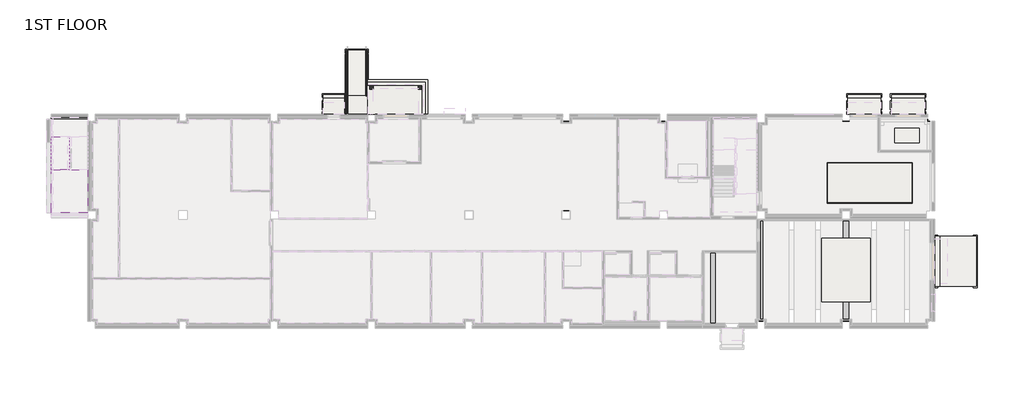
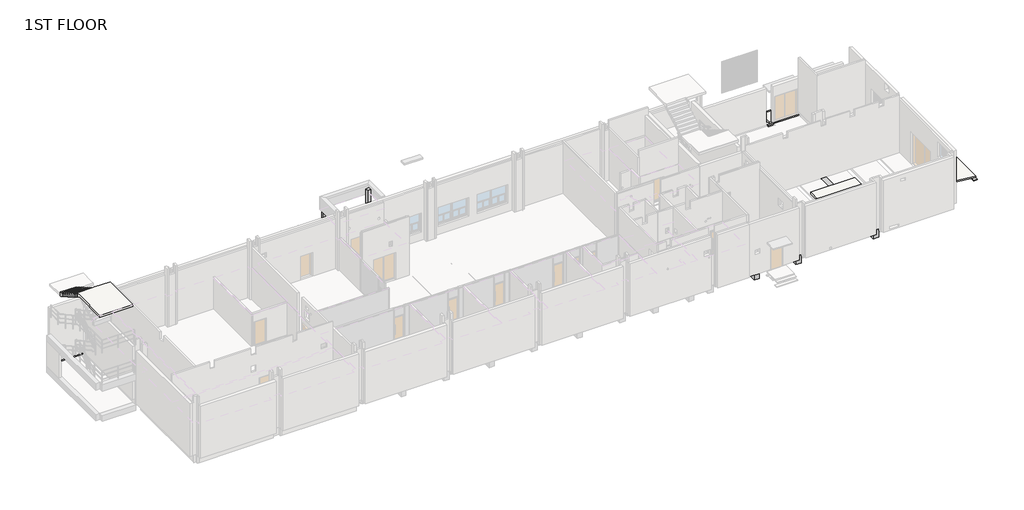
# One storey, part 10 of 15: 37 slabs, 9 beams, 2 columns, 1 stair flight.
"""IFC4 building model written with IfcOpenShell, lengths in millimetres."""

from ifc_helpers import new_model, si_unit, frame, origin, place, context, project, spatial, polyline, outline, extrude, faceted_brep, element, save

model = new_model("IFC4")

# Units and contexts
model_context = context("Model", 3, world=origin())
ifc_project = project(units=[si_unit("LENGTHUNIT", "METRE", prefix="MILLI")], contexts=[model_context])

# Site, building, storey
site = spatial("IfcSite", under=ifc_project)
building = spatial("IfcBuilding", under=site)
storey = spatial("IfcBuildingStorey", under=building, Name="1ST FLOOR", Elevation=4800.0)

# Beams
placement = place(None, origin())
element("IfcBeam", 1, ObjectType="RC Beam_Rectangular : H_SB_AR S16_TG-UG_500x800_1G2A", at=placement, inside=storey, context=model_context, shape_type="Brep", body=[
    faceted_brep([(50825.0, -7850.0, 4800.0), (47350.0, -7850.0, 4800.0), (47350.0, -8350.0, 4800.0), (50825.0, -8350.0, 4800.0), (47350.0, -8350.0, 4650.0), (47350.0, -8350.0, 4000.0), (50825.0, -8350.0, 4000.0), (50825.0, -8350.0, 4650.0), (47350.0, -7850.0, 4000.0), (50825.0, -7850.0, 4000.0), (50825.0, -7850.0, 4650.0), (47350.0, -7850.0, 4650.0)], [[[0, 1, 2, 3]], [[3, 2, 4, 5, 6, 7]], [[8, 9, 6, 5]], [[1, 0, 10, 9, 8, 11]], [[0, 3, 7, 6, 9, 10]], [[8, 5, 4, 2, 1, 11]]]),
])
element("IfcBeam", 2, ObjectType="RC Beam_Rectangular : H_SB_AR S16_TG-UG_500x800_1G1", at=placement, inside=storey, context=model_context, shape_type="Brep", body=[
    faceted_brep([(38750.0, -300.0, 4800.0), (38750.0, -7650.0, 4800.0), (39250.0, -7650.0, 4800.0), (39250.0, -300.0, 4800.0), (39250.0, -7650.0, 4650.0), (39250.0, -7650.0, 4000.0), (39250.0, -300.0, 4000.0), (39250.0, -300.0, 4650.0), (38750.0, -7650.0, 4000.0), (38750.0, -300.0, 4000.0), (38750.0, -300.0, 4650.0), (38750.0, -7650.0, 4650.0)], [[[0, 1, 2, 3]], [[3, 2, 4, 5, 6, 7]], [[6, 5, 8, 9]], [[1, 0, 10, 9, 8, 11]], [[8, 5, 4, 2, 1, 11]], [[0, 3, 7, 6, 9, 10]]]),
])
element("IfcBeam", 3, ObjectType="RC Beam_Rectangular : H_SB_AR S16_TG-UG_500x800_1G1", at=placement, inside=storey, context=model_context, shape_type="Brep", body=[
    faceted_brep([(46800.0, -300.0, 4800.0), (46800.0, -7650.0, 4800.0), (47300.0, -7650.0, 4800.0), (47300.0, -4975.0, 4800.0), (47300.0, -4825.0, 4800.0), (47300.0, -300.0, 4800.0), (47150.0, -300.0, 4800.0), (47300.0, -7650.0, 4000.0), (47300.0, -300.0, 4000.0), (47300.0, -7650.0, 4650.0), (46800.0, -7650.0, 4000.0), (46800.0, -300.0, 4000.0), (46800.0, -300.0, 4650.0), (46800.0, -7650.0, 4650.0)], [[[0, 1, 2, 3, 4, 5, 6]], [[7, 8, 5, 4, 3, 2, 9]], [[8, 7, 10, 11]], [[1, 0, 12, 11, 10, 13]], [[0, 6, 5, 8, 11, 12]], [[10, 7, 9, 2, 1, 13]]]),
])
element("IfcBeam", 4, ObjectType="RC Beam_Rectangular : H_SB_AR S16_TG-UG_450x800_1B1", at=placement, inside=storey, context=model_context, shape_type="Brep", body=[
    faceted_brep([(42125.0, -100.0, 4800.0), (41675.0, -100.0, 4800.0), (41675.0, -7850.0, 4800.0), (42125.0, -7850.0, 4800.0), (42125.0, -7850.0, 4650.0), (42125.0, -7850.0, 4000.0), (42125.0, -100.0, 4000.0), (42125.0, -100.0, 4650.0), (41675.0, -100.0, 4000.0), (41675.0, -7850.0, 4000.0), (41675.0, -100.0, 4650.0), (41675.0, -7850.0, 4650.0)], [[[0, 1, 2, 3]], [[0, 3, 4, 5, 6, 7]], [[8, 6, 5, 9]], [[2, 1, 10, 8, 9, 11]], [[1, 0, 7, 6, 8, 10]], [[3, 2, 11, 9, 5, 4]]]),
])
element("IfcBeam", 5, ObjectType="RC Beam_Rectangular : H_SB_AR S16_TG-UG_450x800_1B1", at=placement, inside=storey, context=model_context, shape_type="Brep", body=[
    faceted_brep([(45325.0, -100.0, 4800.0), (44875.0, -100.0, 4800.0), (44875.0, -7850.0, 4800.0), (45325.0, -7850.0, 4800.0), (45325.0, -7850.0, 4650.0), (45325.0, -7850.0, 4000.0), (45325.0, -100.0, 4000.0), (45325.0, -100.0, 4650.0), (44875.0, -100.0, 4000.0), (44875.0, -7850.0, 4000.0), (44875.0, -100.0, 4650.0), (44875.0, -7850.0, 4650.0)], [[[0, 1, 2, 3]], [[0, 3, 4, 5, 6, 7]], [[8, 6, 5, 9]], [[2, 1, 10, 8, 9, 11]], [[1, 0, 7, 6, 8, 10]], [[3, 2, 11, 9, 5, 4]]]),
])
element("IfcBeam", 6, ObjectType="RC Beam_Rectangular : H_SB_AR S16_TG-UG_450x800_1B1A", at=placement, inside=storey, context=model_context, shape_type="Brep", body=[
    faceted_brep([(50825.0, -8350.0, 4800.0), (51275.0, -8350.0, 4800.0), (51275.0, -8350.0, 4650.0), (51275.0, -8350.0, 4000.0), (50825.0, -8350.0, 4000.0), (50825.0, -8350.0, 4650.0), (50825.0, -16900.0, 4800.0), (51275.0, -16900.0, 4800.0), (51275.0, -16900.0, 4650.0), (51275.0, -16900.0, 4000.0), (50825.0, -16900.0, 4000.0), (50825.0, -15750.0000001, 4000.0), (50825.0, -16900.0, 4650.0)], [[[0, 1, 2, 3, 4, 5]], [[1, 0, 6, 7]], [[1, 7, 8, 9, 3, 2]], [[4, 3, 9, 10, 11]], [[6, 0, 5, 4, 11, 10, 12]], [[7, 6, 12, 10, 9, 8]]]),
])
element("IfcBeam", 7, ObjectType="RC Beam_Rectangular : H_SB_AR S16_TG-UG_500x800_1G1", at=placement, inside=storey, context=model_context, shape_type="Brep", body=[
    faceted_brep([(54700.0, -8350.0, 4800.0), (54700.0, -16700.0, 4800.0), (55200.0, -16700.0, 4800.0), (55200.0, -8350.0, 4800.0), (55200.0, -16700.0, 4650.0), (55200.0, -16700.0, 4000.0), (55200.0, -8350.0, 4000.0), (55200.0, -8350.0, 4650.0), (54700.0, -16700.0, 4000.0), (54700.0, -8350.0, 4000.0), (54700.0, -8350.0, 4650.0), (54700.0, -16700.0, 4650.0)], [[[0, 1, 2, 3]], [[3, 2, 4, 5, 6, 7]], [[6, 5, 8, 9]], [[1, 0, 10, 9, 8, 11]], [[0, 3, 7, 6, 9, 10]], [[8, 5, 4, 2, 1, 11]]]),
])
element("IfcBeam", 8, ObjectType="RC Beam_Rectangular : H_SB_AR S16_TG-UG_500x800_1G1", at=placement, inside=storey, context=model_context, shape_type="Brep", body=[
    faceted_brep([(61750.0, -8350.0, 4800.0), (61750.0, -16700.0, 4800.0), (62250.0, -16700.0, 4800.0), (62250.0, -8350.0, 4800.0), (62250.0, -16700.0, 4650.0), (62250.0, -16700.0, 4000.0), (62250.0, -8350.0, 4000.0), (62250.0, -8350.0, 4650.0), (61750.0, -16700.0, 4000.0), (61750.0, -8350.0, 4000.0), (61750.0, -8350.0, 4650.0), (61750.0, -16700.0, 4650.0)], [[[0, 1, 2, 3]], [[3, 2, 4, 5, 6, 7]], [[6, 5, 8, 9]], [[1, 0, 10, 9, 8, 11]], [[0, 3, 7, 6, 9, 10]], [[8, 5, 4, 2, 1, 11]]]),
])
element("IfcBeam", 9, ObjectType="RC Beam_Rectangular : H_SB_AR S16_RC Beam-AG_400x530_SG1A", at=placement, inside=storey, context=model_context, shape_type="Brep", body=[
    faceted_brep([(-300.0, -100.0, 4630.0), (-300.0, 50.0, 4630.0), (-300.0, 300.0, 4630.0), (-3300.0, 300.0, 4630.0), (-3300.0, 50.0, 4630.0), (-3300.0, -100.0, 4630.0), (-300.0, -100.0, 4100.0), (-300.0, -100.0, 4430.0), (-3300.0, -100.0, 4430.0), (-3300.0, -100.0, 4100.0), (-300.0, 300.0, 4100.0), (-3300.0, 300.0, 4100.0)], [[[0, 1, 2, 3, 4, 5]], [[6, 7, 0, 5, 8, 9]], [[10, 6, 9, 11]], [[2, 10, 11, 3]], [[2, 1, 0, 7, 6, 10]], [[3, 11, 9, 8, 5, 4]]]),
])

# Columns
element("IfcColumn", 10, ObjectType="RC_Column_Rectangular : H_SC_AR S15_RC Col-AG_300x300_C4", at=placement, inside=storey, context=model_context, shape_type="Brep", body=[
    faceted_brep([(23150.0, 2650.0, 4585.0), (23150.0, 2620.0, 4585.0), (23150.0, 2350.0, 4585.0), (22850.0, 2350.0, 4585.0), (22850.0, 2620.0, 4585.0), (22850.0, 2650.0, 4585.0), (23150.0, 2650.0, 9300.0), (23150.0, 2350.0, 9300.0), (23150.0, 2350.0, 4750.0), (22850.0, 2350.0, 9300.0), (22850.0, 2350.0, 4750.0), (22850.0, 2650.0, 9300.0), (23000.0, 2650.0, 9300.0)], [[[0, 1, 2, 3, 4, 5]], [[6, 7, 8, 2, 1, 0]], [[7, 9, 10, 3, 2, 8]], [[9, 11, 5, 4, 3, 10]], [[11, 12, 6, 0, 5]], [[6, 12, 11, 9, 7]]]),
])
element("IfcColumn", 11, ObjectType="RC_Column_Rectangular : H_SC_AR S15_RC Col-AG_300x300_C4", at=placement, inside=storey, context=model_context, shape_type="Brep", body=[
    faceted_brep([(27150.0, 2650.0, 4585.0), (27150.0, 2350.0, 4585.0), (27120.0, 2350.0, 4585.0), (26850.0, 2350.0, 4585.0), (26850.0, 2620.0, 4585.0), (26850.0, 2650.0, 4585.0), (27150.0, 2650.0, 9300.0), (27150.0, 2500.0, 9300.0), (27150.0, 2350.0, 9300.0), (26850.0, 2350.0, 9300.0), (26850.0, 2350.0, 4750.0), (26850.0, 2650.0, 9300.0)], [[[0, 1, 2, 3, 4, 5]], [[6, 7, 8, 1, 0]], [[8, 9, 10, 3, 2, 1]], [[9, 11, 5, 4, 3, 10]], [[11, 6, 0, 5]], [[6, 11, 9, 8, 7]]]),
])

# Slabs
element("IfcSlab", 12, ObjectType="H_SF_AR S18_MAT_T650_MF2", at=placement, inside=storey, context=model_context, shape_type="Brep", body=[
    faceted_brep([(27625.0, 3125.0000075, 4100.0), (27625.0, 300.0, 4100.0), (22650.0, 300.0, 4100.0), (22650.0, 3125.0000075, 4100.0), (22650.0, 300.0, 4750.0), (27120.0, 300.0, 4750.0), (27120.0, 2350.0, 4750.0), (26850.0, 2350.0, 4750.0), (26850.0, 2620.0, 4750.0), (23150.0, 2620.0, 4750.0), (23150.0, 2350.0, 4750.0), (22850.0, 2350.0, 4750.0), (22850.0, 2620.0, 4750.0), (22650.0, 2620.0, 4750.0), (27625.0, 3125.0000075, 4500.0), (27625.0, 300.0, 4500.0), (27420.0, 300.0, 4500.0), (27420.0, 300.0, 4585.0), (27120.0, 300.0, 4585.0), (22650.0, 300.0, 4500.0), (22650.0, 300.0, 4450.0), (22650.0, 300.0, 4400.0), (22650.0, 2620.0, 4585.0), (22650.0, 2920.0, 4585.0), (22650.0, 2920.0, 4500.0), (22650.0, 3125.0000075, 4500.0), (22650.0, 3125.0000075, 4361.6666662), (22650.0, 3125.0000075, 4311.5556782), (27420.0, 2920.0, 4585.0), (22850.0, 2620.0, 4585.0), (22850.0, 2350.0, 4585.0), (23150.0, 2350.0, 4585.0), (23150.0, 2620.0, 4585.0), (26850.0, 2620.0, 4585.0), (26850.0, 2350.0, 4585.0), (27120.0, 2350.0, 4585.0), (27420.0, 2920.0, 4500.0)], [[[0, 1, 2, 3]], [[4, 5, 6, 7, 8, 9, 10, 11, 12, 13]], [[1, 0, 14, 15]], [[2, 1, 15, 16, 17, 18, 5, 4, 19, 20, 21]], [[3, 2, 21, 20, 19, 4, 13, 22, 23, 24, 25, 26, 27]], [[0, 3, 27, 26, 25, 14]], [[17, 28, 23, 22, 29, 30, 31, 32, 33, 34, 35, 18]], [[28, 17, 16, 36]], [[36, 16, 15, 14, 25, 24]], [[5, 18, 35, 6]], [[23, 28, 36, 24]], [[8, 33, 32, 9]], [[22, 13, 12, 29]], [[35, 34, 7, 6]], [[34, 33, 8, 7]], [[32, 31, 10, 9]], [[31, 30, 11, 10]], [[30, 29, 12, 11]]]),
])
element("IfcSlab", 13, ObjectType="H_SF_AR B01_EQ Fdn_T800_EF1", at=placement, inside=storey, context=model_context, shape_type="Brep", body=[
    faceted_brep([(60500.0, -3750.0, 4200.0), (67400.0, -3750.0, 4200.0), (67400.0, -6950.0, 4200.0), (60500.0, -6950.0, 4200.0), (60500.0, -3750.0, 5000.0), (60500.0, -6950.0, 5000.0), (67400.0, -6950.0, 5000.0), (67400.0, -3750.0, 5000.0), (60500.0, -3750.0, 4600.0), (60500.0, -3750.0, 4650.0), (67400.0, -3750.0, 4650.0), (67400.0, -3750.0, 4600.0), (67400.0, -6950.0, 4650.0), (67400.0, -6950.0, 4600.0), (60500.0, -6950.0, 4650.0), (60500.0, -6950.0, 4600.0)], [[[0, 1, 2, 3]], [[4, 5, 6, 7]], [[1, 0, 8, 9, 4, 7, 10, 11]], [[2, 1, 11, 10, 7, 6, 12, 13]], [[3, 2, 13, 12, 6, 5, 14, 15]], [[0, 3, 15, 14, 5, 4, 9, 8]]]),
])
element("IfcSlab", 14, ObjectType="H_SF_AR B01_EQ Fdn_T200_EF2", at=placement, inside=storey, context=model_context, shape_type="SweptSolid", body=[
    extrude(outline(polyline([(64000.0000005, -9900.0), (64000.0000005, -15100.0), (59999.9999995, -15100.0), (59999.9999995, -9900.0), (64000.0000005, -9900.0)])), frame((0.0, 0.0, 4800.0), z_axis=(0.0, 0.0, 1.0), x_axis=(1.0, 0.0, 0.0)), (0.0, 0.0, 1.0), 200.0),
])
element("IfcSlab", 15, ObjectType="H_SF_AR B01_EQ Fdn_T200_EF3", at=placement, inside=storey, context=model_context, shape_type="SweptSolid", body=[
    extrude(outline(polyline([(66000.0, -850.0), (68000.0, -850.0), (68000.0, -2050.0), (66000.0, -2050.0), (66000.0, -850.0)])), frame((0.0, 0.0, 4800.0), z_axis=(0.0, 0.0, 1.0), x_axis=(1.0, 0.0, 0.0)), (0.0, 0.0, 1.0), 200.0),
])
element("IfcSlab", 16, ObjectType="H_FL_AR_S17_RC Slab_T200_SS1", at=placement, inside=storey, context=model_context, shape_type="Brep", body=[
    faceted_brep([(-1850.0, -4250.0, 14050.0), (-3300.0, -4250.0, 14050.0), (-3300.0, -4604.0698283, 14050.0), (-3300.0, -7800.0, 14050.0), (-300.0, -7800.0, 14050.0), (-300.0, -4250.0, 14050.0), (-1750.0, -4250.0, 14050.0), (-1850.0, -4250.0, 13850.0), (-1850.0, -4250.0, 13643.4592668), (-3300.0, -4250.0, 13643.4592668), (-3300.0, -4604.0698283, 13850.0), (-3300.0, -7800.0, 13850.0), (-300.0, -7800.0, 13850.0), (-300.0, -4250.0, 13850.0), (-1750.0, -4250.0, 13850.0), (-1850.0, -4604.0698283, 13850.0)], [[[0, 1, 2, 3, 4, 5, 6]], [[1, 0, 7, 8, 9]], [[1, 9, 10, 11, 3, 2]], [[4, 3, 11, 12]], [[5, 4, 12, 13]], [[0, 6, 14, 7]], [[10, 15, 7, 14, 13, 12, 11]], [[15, 10, 9, 8]], [[7, 15, 8]], [[6, 5, 13, 14]]]),
])
element("IfcSlab", 17, ObjectType="H_SF_AR_B08_Ramp_T150", at=placement, inside=storey, context=model_context, shape_type="SweptSolid", body=[
    extrude(outline(polyline([(69700.0, -9750.0), (69700.0, -13850.0), (69312.0, -13850.0), (69312.0, -9750.0), (69700.0, -9750.0)])), frame((0.0, 0.0, 4650.0), z_axis=(0.0, 0.0, 1.0), x_axis=(1.0, 0.0, 0.0)), (0.0, 0.0, 1.0), 150.0),
])
element("IfcSlab", 18, ObjectType="H_SF_AR_B08_Ramp_T150", at=placement, inside=storey, context=model_context, shape_type="Brep", body=[
    faceted_brep([(72700.0, -9750.0, 4349.2518657), (72700.0, -10050.0, 4349.2518657), (72700.0, -13550.0, 4349.2518657), (72700.0, -13850.0, 4349.2518657), (72256.3868159, -13850.0, 4393.6131841), (72256.3868159, -13550.0, 4393.6131841), (72256.3868159, -10050.0, 4393.6131841), (72256.3868159, -9750.0, 4393.6131841), (69700.0, -10050.0, 4649.2518657), (69700.0, -9750.0, 4649.2518657), (72250.0, -9750.0, 4394.2518657), (72250.0, -10050.0, 4394.2518657), (72250.0, -13550.0, 4394.2518657), (72250.0, -13850.0, 4394.2518657), (69700.0, -13850.0, 4649.2518657), (69700.0, -13550.0, 4649.2518657), (72700.0, -13850.0, 4500.0), (72700.0, -9750.0, 4500.0), (69700.0, -9750.0, 4800.0), (69700.0, -13850.0, 4800.0), (69700.0, -13850.0, 4650.0), (72250.0, -13850.0, 4400.0), (69700.0, -9750.0, 4650.0), (72250.0, -9750.0, 4400.0)], [[[0, 1, 2, 3, 4, 5, 6, 7]], [[8, 9, 10, 11, 12, 13, 14, 15]], [[16, 17, 18, 19]], [[17, 16, 3, 2, 1, 0]], [[16, 19, 20, 14, 13, 21, 4, 3]], [[19, 18, 22, 9, 8, 15, 14, 20]], [[18, 17, 0, 7, 23, 10, 9, 22]], [[21, 23, 7, 6, 5, 4]], [[23, 21, 13, 12, 11, 10]]]),
])
element("IfcSlab", 19, ObjectType="H_SF_AR_S18_Lean_T50", at=placement, inside=storey, context=model_context, shape_type="SweptSolid", body=[
    extrude(outline(polyline([(69550.0, -9650.0), (69550.0, -13950.0), (69300.0, -13950.0), (69300.0, -9650.0), (69550.0, -9650.0)])), frame((0.0, 0.0, 4450.0), z_axis=(0.0, 0.0, 1.0), x_axis=(1.0, 0.0, 0.0)), (0.0, 0.0, 1.0), 50.0),
])
element("IfcSlab", 20, ObjectType="H_SF_AR_S18_Lean_T50", at=placement, inside=storey, context=model_context, shape_type="SweptSolid", body=[
    extrude(outline(polyline([(72450.0, -9650.0), (72800.0, -9650.0), (72800.0, -13950.0), (72450.0, -13950.0), (72450.0, -9650.0)])), frame((0.0, 0.0, 4150.0), z_axis=(0.0, 0.0, 1.0), x_axis=(1.0, 0.0, 0.0)), (0.0, 0.0, 1.0), 50.0),
])
element("IfcSlab", 21, ObjectType="H_SF_AR_S18_Lean_T50", at=placement, inside=storey, context=model_context, shape_type="Brep", body=[
    faceted_brep([(69700.0, -13550.0, 4599.0024876), (69700.0, -10050.0, 4599.0024876), (69717.9210597, -10050.0, 4597.2103816), (72233.6520381, -10050.0, 4345.6372838), (72233.6520381, -13550.0, 4345.6372838), (69717.9210597, -13550.0, 4597.2103816), (69700.0, -10050.0, 4649.2518657), (69700.0, -13550.0, 4649.2518657), (72250.0, -13550.0, 4394.2518657), (72250.0, -10050.0, 4394.2518657), (69700.0, -13550.0, 4600.0), (72229.2893219, -13550.0, 4350.0), (72250.0, -13550.0, 4350.0), (69700.0, -10050.0, 4600.0), (72250.0, -10050.0, 4350.0), (72229.2893219, -10050.0, 4350.0)], [[[0, 1, 2, 3, 4, 5]], [[6, 7, 8, 9]], [[7, 10, 0, 5, 4, 11, 12, 8]], [[1, 0, 10, 7, 6, 13]], [[1, 13, 6, 9, 14, 15, 3, 2]], [[15, 11, 4, 3]], [[11, 15, 14, 12]], [[12, 14, 9, 8]]]),
])
element("IfcSlab", 22, ObjectType="H_SF_AR_B08_Ramp_T150", at=placement, inside=storey, context=model_context, shape_type="Brep", body=[
    faceted_brep([(22638.0, 1800.0, 4600.0), (22638.0, 312.0, 4600.0), (22338.0, 312.0, 4600.0), (21238.0, 312.0, 4600.0), (20938.0, 312.0, 4600.0), (20938.0, 1800.0, 4600.0), (22638.0, 1800.0, 4750.0), (20938.0, 1800.0, 4750.0), (20938.0, 312.0, 4750.0), (22638.0, 312.0, 4750.0)], [[[0, 1, 2, 3, 4, 5]], [[6, 7, 8, 9]], [[1, 0, 6, 9]], [[4, 3, 2, 1, 9, 8]], [[5, 4, 8, 7]], [[0, 5, 7, 6]]]),
])
element("IfcSlab", 23, ObjectType="H_SF_AR_B08_Stoop_T150", at=placement, inside=storey, context=model_context, shape_type="Brep", body=[
    faceted_brep([(68450.0, 1600.0, 4600.0), (68450.0, 1400.0, 4600.0), (68450.0, 662.0000074, 4600.0), (68450.0, 312.0000074, 4600.0), (65750.0, 312.0000074, 4600.0), (65750.0, 662.0000074, 4600.0), (65750.0, 1400.0, 4600.0), (65750.0, 1600.0, 4600.0), (68450.0, 1600.0, 4750.0), (65750.0, 1600.0, 4750.0), (65750.0, 312.0000074, 4750.0), (68450.0, 312.0000074, 4750.0), (68450.0, 1600.0, 4625.0), (65750.0, 1600.0, 4625.0)], [[[0, 1, 2, 3, 4, 5, 6, 7]], [[8, 9, 10, 11]], [[3, 2, 1, 0, 12, 8, 11]], [[4, 3, 11, 10]], [[7, 6, 5, 4, 10, 9, 13]], [[0, 7, 13, 9, 8, 12]]]),
])
element("IfcSlab", 24, ObjectType="H_SF_AR_B08_Stoop_T125", at=placement, inside=storey, context=model_context, shape_type="SweptSolid", body=[
    extrude(outline(polyline([(68450.0, 1900.0), (68450.0, 1600.0), (65750.0, 1600.0), (65750.0, 1900.0), (68450.0, 1900.0)])), frame((0.0, 0.0, 4600.0), z_axis=(0.0, 0.0, 1.0), x_axis=(1.0, 0.0, 0.0)), (0.0, 0.0, 1.0), 25.0),
])
element("IfcSlab", 25, ObjectType="H_SF_AR_S18_Lean_T50", at=placement, inside=storey, context=model_context, shape_type="SweptSolid", body=[
    extrude(outline(polyline([(68550.0, 2000.0), (68550.0, 1700.0), (65650.0, 1700.0), (65650.0, 2000.0), (68550.0, 2000.0)])), frame((0.0, 0.0, 4250.0), z_axis=(0.0, 0.0, 1.0), x_axis=(1.0, 0.0, 0.0)), (0.0, 0.0, 1.0), 50.0),
])
element("IfcSlab", 26, ObjectType="H_SF_AR_S18_Lean_T50", at=placement, inside=storey, context=model_context, shape_type="SweptSolid", body=[
    extrude(outline(polyline([(68550.0, 300.0), (65650.0, 300.0), (65650.0, 512.0000074), (68550.0, 512.0000074), (68550.0, 300.0)])), frame((0.0, 0.0, 4400.0), z_axis=(0.0, 0.0, 1.0), x_axis=(1.0, 0.0, 0.0)), (0.0, 0.0, 1.0), 50.0),
])
element("IfcSlab", 27, ObjectType="H_SF_AR_S18_Lean_T50", at=placement, inside=storey, context=model_context, shape_type="Brep", body=[
    faceted_brep([(68550.0, 1400.0, 4550.0), (68550.0, 1379.2893219, 4550.0), (68550.0, 682.7106855, 4550.0), (68550.0, 662.0000074, 4550.0), (65650.0, 662.0000074, 4550.0), (65650.0, 682.7106855, 4550.0), (65650.0, 1379.2893219, 4550.0), (65650.0, 1400.0, 4550.0), (68550.0, 1400.0, 4600.0), (65650.0, 1400.0, 4600.0), (65650.0, 662.0000074, 4600.0), (68550.0, 662.0000074, 4600.0)], [[[0, 1, 2, 3, 4, 5, 6, 7]], [[8, 9, 10, 11]], [[3, 2, 1, 0, 8, 11]], [[4, 3, 11, 10]], [[7, 6, 5, 4, 10, 9]], [[0, 7, 9, 8]]]),
])
element("IfcSlab", 28, ObjectType="H_SF_AR_B08_Stoop_T150", at=placement, inside=storey, context=model_context, shape_type="Brep", body=[
    faceted_brep([(64850.0, 1600.0, 4600.0), (64850.0, 1400.0, 4600.0), (64850.0, 662.0000074, 4600.0), (64850.0, 312.0000074, 4600.0), (62150.0, 312.0000074, 4600.0), (62150.0, 662.0000074, 4600.0), (62150.0, 1400.0, 4600.0), (62150.0, 1600.0, 4600.0), (64850.0, 1600.0, 4750.0), (62150.0, 1600.0, 4750.0), (62150.0, 312.0000074, 4750.0), (64850.0, 312.0000074, 4750.0), (64850.0, 1600.0, 4625.0), (62150.0, 1600.0, 4625.0)], [[[0, 1, 2, 3, 4, 5, 6, 7]], [[8, 9, 10, 11]], [[3, 2, 1, 0, 12, 8, 11]], [[4, 3, 11, 10]], [[7, 6, 5, 4, 10, 9, 13]], [[0, 7, 13, 9, 8, 12]]]),
])
element("IfcSlab", 29, ObjectType="H_SF_AR_B08_Stoop_T125", at=placement, inside=storey, context=model_context, shape_type="SweptSolid", body=[
    extrude(outline(polyline([(64850.0, 1900.0), (64850.0, 1600.0), (62150.0, 1600.0), (62150.0, 1900.0), (64850.0, 1900.0)])), frame((0.0, 0.0, 4600.0), z_axis=(0.0, 0.0, 1.0), x_axis=(1.0, 0.0, 0.0)), (0.0, 0.0, 1.0), 25.0),
])
element("IfcSlab", 30, ObjectType="H_SF_AR_S18_Lean_T50", at=placement, inside=storey, context=model_context, shape_type="SweptSolid", body=[
    extrude(outline(polyline([(64950.0, 2000.0), (64950.0, 1700.0), (62050.0, 1700.0), (62050.0, 2000.0), (64950.0, 2000.0)])), frame((0.0, 0.0, 4250.0), z_axis=(0.0, 0.0, 1.0), x_axis=(1.0, 0.0, 0.0)), (0.0, 0.0, 1.0), 50.0),
])
element("IfcSlab", 31, ObjectType="H_SF_AR_S18_Lean_T50", at=placement, inside=storey, context=model_context, shape_type="SweptSolid", body=[
    extrude(outline(polyline([(64950.0, 300.0), (62050.0, 300.0), (62050.0, 512.0000074), (64950.0, 512.0000074), (64950.0, 300.0)])), frame((0.0, 0.0, 4400.0), z_axis=(0.0, 0.0, 1.0), x_axis=(1.0, 0.0, 0.0)), (0.0, 0.0, 1.0), 50.0),
])
element("IfcSlab", 32, ObjectType="H_SF_AR_S18_Lean_T50", at=placement, inside=storey, context=model_context, shape_type="Brep", body=[
    faceted_brep([(64950.0, 1400.0, 4550.0), (64950.0, 1379.2893219, 4550.0), (64950.0, 682.7106855, 4550.0), (64950.0, 662.0000074, 4550.0), (62050.0, 662.0000074, 4550.0), (62050.0, 682.7106855, 4550.0), (62050.0, 1379.2893219, 4550.0), (62050.0, 1400.0, 4550.0), (64950.0, 1400.0, 4600.0), (62050.0, 1400.0, 4600.0), (62050.0, 662.0000074, 4600.0), (64950.0, 662.0000074, 4600.0)], [[[0, 1, 2, 3, 4, 5, 6, 7]], [[8, 9, 10, 11]], [[3, 2, 1, 0, 8, 11]], [[4, 3, 11, 10]], [[7, 6, 5, 4, 10, 9]], [[0, 7, 9, 8]]]),
])
element("IfcSlab", 33, ObjectType="H_SF_AR_B08_Stoop_T150", at=placement, inside=storey, context=model_context, shape_type="Brep", body=[
    faceted_brep([(20750.0, 1600.0, 4630.0), (20750.0, 1400.0, 4630.0), (20750.0, 662.0000074, 4630.0), (20750.0, 312.0000074, 4630.0), (19050.0, 312.0000074, 4630.0), (19050.0, 662.0000074, 4630.0), (19050.0, 1400.0, 4630.0), (19050.0, 1600.0, 4630.0), (20750.0, 1600.0, 4780.0), (19050.0, 1600.0, 4780.0), (19050.0, 312.0000074, 4780.0), (20750.0, 312.0000074, 4780.0), (20750.0, 1600.0, 4640.0), (19050.0, 1600.0, 4640.0)], [[[0, 1, 2, 3, 4, 5, 6, 7]], [[8, 9, 10, 11]], [[3, 2, 1, 0, 12, 8, 11]], [[4, 3, 11, 10]], [[7, 6, 5, 4, 10, 9, 13]], [[0, 7, 13, 9, 8, 12]]]),
])
element("IfcSlab", 34, ObjectType="H_SF_AR_B08_Stoop_T125", at=placement, inside=storey, context=model_context, shape_type="Brep", body=[
    faceted_brep([(20750.0, 1900.0, 4515.0), (20750.0, 1600.0, 4515.0), (19050.0, 1600.0, 4515.0), (19050.0, 1900.0, 4515.0), (20750.0, 1900.0, 4640.0), (19050.0, 1900.0, 4640.0), (19050.0, 1600.0, 4640.0), (20750.0, 1600.0, 4640.0), (20750.0, 1600.0, 4630.0), (19050.0, 1600.0, 4630.0)], [[[0, 1, 2, 3]], [[4, 5, 6, 7]], [[1, 0, 4, 7, 8]], [[2, 1, 8, 7, 6, 9]], [[3, 2, 9, 6, 5]], [[0, 3, 5, 4]]]),
])
element("IfcSlab", 35, ObjectType="H_SF_AR_S18_Lean_T50", at=placement, inside=storey, context=model_context, shape_type="SweptSolid", body=[
    extrude(outline(polyline([(20850.0, 2000.0), (20850.0, 1700.0), (18950.0, 1700.0), (18950.0, 2000.0), (20850.0, 2000.0)])), frame((0.0, 0.0, 4280.0), z_axis=(0.0, 0.0, 1.0), x_axis=(1.0, 0.0, 0.0)), (0.0, 0.0, 1.0), 50.0),
])
element("IfcSlab", 36, ObjectType="H_SF_AR_S18_Lean_T50", at=placement, inside=storey, context=model_context, shape_type="Brep", body=[
    faceted_brep([(20850.0, 300.0, 4430.0), (18950.0, 300.0, 4430.0), (18950.0, 512.0000074, 4430.0), (20850.0, 512.0000074, 4430.0), (20850.0, 300.0, 4480.0), (20850.0, 512.0000074, 4480.0), (18950.0, 512.0000074, 4480.0), (18950.0, 300.0, 4480.0), (20850.0, 300.0, 4450.0)], [[[0, 1, 2, 3]], [[4, 5, 6, 7]], [[1, 0, 8, 4, 7]], [[2, 1, 7, 6]], [[3, 2, 6, 5]], [[0, 3, 5, 4, 8]]]),
])
element("IfcSlab", 37, ObjectType="H_SF_AR_S18_Lean_T50", at=placement, inside=storey, context=model_context, shape_type="Brep", body=[
    faceted_brep([(20850.0, 1400.0, 4580.0), (20850.0, 1379.2893219, 4580.0), (20850.0, 682.7106855, 4580.0), (20850.0, 662.0000074, 4580.0), (18950.0, 662.0000074, 4580.0), (18950.0, 682.7106855, 4580.0), (18950.0, 1379.2893219, 4580.0), (18950.0, 1400.0, 4580.0), (20850.0, 1400.0, 4630.0), (18950.0, 1400.0, 4630.0), (18950.0, 662.0000074, 4630.0), (20850.0, 662.0000074, 4630.0)], [[[0, 1, 2, 3, 4, 5, 6, 7]], [[8, 9, 10, 11]], [[3, 2, 1, 0, 8, 11]], [[4, 3, 11, 10]], [[7, 6, 5, 4, 10, 9]], [[0, 7, 9, 8]]]),
])
element("IfcSlab", 38, ObjectType="H_SF_AR_B08_Ramp_T150", at=placement, inside=storey, context=model_context, shape_type="Brep", body=[
    faceted_brep([(22638.0, 5550.0, 4349.6670362), (22638.0, 5100.0, 4379.6670362), (22638.0, 1800.0, 4599.6670362), (22338.0, 1800.0, 4599.6670362), (21238.0, 1800.0, 4599.6670362), (20938.0, 1800.0, 4599.6670362), (20938.0, 5100.0, 4379.6670362), (20938.0, 5550.0, 4349.6670362), (22638.0, 5550.0, 4500.0), (20938.0, 5550.0, 4500.0), (20938.0, 1800.0, 4750.0), (22638.0, 1800.0, 4750.0), (22638.0, 1800.0, 4600.0), (20938.0, 1800.0, 4600.0)], [[[0, 1, 2, 3, 4, 5, 6, 7]], [[8, 9, 10, 11]], [[2, 1, 0, 8, 11, 12]], [[5, 4, 3, 2, 12, 11, 10, 13]], [[7, 6, 5, 13, 10, 9]], [[0, 7, 9, 8]]]),
])
element("IfcSlab", 39, ObjectType="H_SF_AR_S18_Lean_T50", at=placement, inside=storey, context=model_context, shape_type="SweptSolid", body=[
    extrude(outline(polyline([(22488.0, 300.0), (21088.0, 300.0), (21088.0, 550.0), (22488.0, 550.0), (22488.0, 300.0)])), frame((0.0, 0.0, 4400.0), z_axis=(0.0, 0.0, 1.0), x_axis=(1.0, 0.0, 0.0)), (0.0, 0.0, 1.0), 50.0),
])
element("IfcSlab", 40, ObjectType="H_SF_AR_S18_Lean_T50", at=placement, inside=storey, context=model_context, shape_type="SweptSolid", body=[
    extrude(outline(polyline([(22738.0, 5650.0), (22738.0, 5300.0), (20838.0, 5300.0), (20838.0, 5650.0), (22738.0, 5650.0)])), frame((0.0, 0.0, 4129.6670362), z_axis=(0.0, 0.0, 1.0), x_axis=(1.0, 0.0, 0.0)), (0.0, 0.0, 1.0), 50.0),
])
element("IfcSlab", 41, ObjectType="H_SF_AR_S18_Lean_T50", at=placement, inside=storey, context=model_context, shape_type="Brep", body=[
    faceted_brep([(22338.0, 1800.0, 4550.0), (22338.0, 700.0, 4550.0), (21238.0, 700.0, 4550.0), (21238.0, 1800.0, 4550.0), (22338.0, 1800.0, 4600.0), (21238.0, 1800.0, 4600.0), (21238.0, 700.0, 4600.0), (22338.0, 700.0, 4600.0), (22338.0, 1800.0, 4599.6670362), (21238.0, 1800.0, 4599.6670362)], [[[0, 1, 2, 3]], [[4, 5, 6, 7]], [[1, 0, 8, 4, 7]], [[2, 1, 7, 6]], [[3, 2, 6, 5, 9]], [[0, 3, 9, 5, 4, 8]]]),
])
element("IfcSlab", 42, ObjectType="H_SF_AR_S18_Lean_T50", at=placement, inside=storey, context=model_context, shape_type="Brep", body=[
    faceted_brep([(20850.0, 1800.0, 4400.0), (21088.0, 1800.0, 4400.0), (21088.0, 550.0, 4400.0), (21088.0, 300.0, 4400.0), (20850.0, 300.0, 4400.0), (21088.0, 1800.0, 4450.0), (20850.0, 1800.0, 4450.0), (20850.0, 300.0, 4450.0), (21088.0, 300.0, 4450.0), (21088.0, 550.0, 4450.0), (20850.0, 300.0, 4430.0)], [[[0, 1, 2, 3, 4]], [[5, 6, 7, 8, 9]], [[1, 0, 6, 5]], [[1, 5, 9, 8, 3, 2]], [[4, 3, 8, 7, 10]], [[0, 4, 10, 7, 6]]]),
    faceted_brep([(22650.0, 1800.0, 4400.0), (22650.0, 300.0, 4400.0), (22488.0, 300.0, 4400.0), (22488.0, 550.0, 4400.0), (22488.0, 1800.0, 4400.0), (22650.0, 300.0, 4450.0), (22650.0, 1800.0, 4450.0), (22488.0, 1800.0, 4450.0), (22488.0, 550.0, 4450.0), (22488.0, 300.0, 4450.0)], [[[0, 1, 2, 3, 4]], [[5, 6, 7, 8, 9]], [[1, 0, 6, 5]], [[2, 1, 5, 9]], [[2, 9, 8, 7, 4, 3]], [[0, 4, 7, 6]]]),
])
element("IfcSlab", 43, ObjectType="H_SF_AR_S18_Lean_T50", at=placement, inside=storey, context=model_context, shape_type="Brep", body=[
    faceted_brep([(22738.0, 5238.2864422, 4170.6699159), (22738.0, 3125.0000075, 4311.5556782), (22650.0, 3125.0000075, 4311.5556782), (22650.0, 1800.0, 4399.8890121), (22488.0, 1800.0, 4399.8890121), (22488.0, 5238.2864422, 4170.6699159), (22488.0, 1800.0, 4450.0), (22650.0, 1800.0, 4450.0), (22650.0, 3125.0000075, 4361.6666662), (22738.0, 3125.0000075, 4361.6666662), (22738.0, 5184.596098, 4224.3602601), (22638.0, 5184.596098, 4224.3602601), (22488.0, 5184.596098, 4224.3602601)], [[[0, 1, 2, 3, 4, 5]], [[6, 7, 8, 9, 10, 11, 12]], [[1, 0, 10, 9]], [[4, 3, 7, 6]], [[5, 4, 6, 12]], [[0, 5, 12, 11, 10]], [[2, 1, 9, 8]], [[3, 2, 8, 7]]]),
    faceted_brep([(21088.0, 1800.0, 4399.8890121), (20850.0, 1800.0, 4399.8890121), (20850.0, 5238.2864422, 4170.6699159), (21088.0, 5238.2864422, 4170.6699159), (20850.0, 1800.0, 4450.0), (21088.0, 1800.0, 4450.0), (21088.0, 5184.596098, 4224.3602601), (20938.0, 5184.596098, 4224.3602601), (20850.0, 5184.596098, 4224.3602601)], [[[0, 1, 2, 3]], [[4, 5, 6, 7, 8]], [[1, 0, 5, 4]], [[2, 1, 4, 8]], [[0, 3, 6, 5]], [[3, 2, 8, 7, 6]]]),
])
element("IfcSlab", 44, ObjectType="H_SF_AR_S18_Lean_T50", at=placement, inside=storey, context=model_context, shape_type="Brep", body=[
    faceted_brep([(65557.0, -1062.0, 4600.0), (65557.0, -100.0, 4600.0), (65577.7106781, -100.0, 4600.0), (68700.0, -100.0, 4600.0), (68700.0, -300.0, 4600.0), (68900.0, -300.0, 4600.0), (68900.0, -2372.2893219, 4600.0), (68900.0, -2393.0, 4600.0), (65057.0, -2393.0, 4600.0), (65057.0, -1082.7106781, 4600.0), (65057.0, -1062.0, 4600.0), (65077.7106781, -1062.0, 4600.0), (65057.0, -1062.0, 4650.0), (65057.0, -2393.0, 4650.0), (68900.0, -2393.0, 4650.0), (68900.0, -300.0, 4650.0), (68700.0, -300.0, 4650.0), (68700.0, -100.0, 4650.0), (65557.0, -100.0, 4650.0), (65557.0, -1062.0, 4650.0)], [[[0, 1, 2, 3, 4, 5, 6, 7, 8, 9, 10, 11]], [[12, 13, 14, 15, 16, 17, 18, 19]], [[13, 12, 10, 9, 8]], [[12, 19, 0, 11, 10]], [[1, 0, 19, 18]], [[18, 17, 3, 2, 1]], [[4, 3, 17, 16]], [[5, 4, 16, 15]], [[15, 14, 7, 6, 5]], [[8, 7, 14, 13]]]),
])
element("IfcSlab", 45, ObjectType="H_SF_AR_S18_Lean_T50", at=placement, inside=storey, context=model_context, shape_type="Brep", body=[
    faceted_brep([(64357.0, -3093.0, 4600.0), (68900.0, -3093.0, 4600.0), (68900.0, -3113.7106781, 4600.0), (68900.0, -7650.0, 4600.0), (68600.0, -7650.0, 4600.0), (68600.0, -7950.0, 4600.0), (62350.0, -7950.0, 4600.0), (62350.0, -7650.0, 4600.0), (61650.0, -7650.0, 4600.0), (61650.0, -7950.0, 4600.0), (55350.0, -7950.0, 4600.0), (55350.0, -7650.0, 4600.0), (55050.0, -7650.0, 4600.0), (55050.0, -400.0, 4600.0), (55350.0, -400.0, 4600.0), (55350.0, -100.0, 4600.0), (61700.0, -100.0, 4600.0), (61700.0, -300.0, 4600.0), (62300.0, -300.0, 4600.0), (62300.0, -100.0, 4600.0), (64357.0, -100.0, 4600.0), (64357.0, -912.0, 4600.0), (64357.0, -1062.0, 4600.0), (64357.0, -1082.7106781, 4600.0), (67400.0, -3750.0, 4600.0), (60500.0, -3750.0, 4600.0), (60500.0, -6950.0, 4600.0), (67400.0, -6950.0, 4600.0), (68900.0, -3093.0, 4650.0), (64357.0, -3093.0, 4650.0), (64357.0, -912.0, 4650.0), (64357.0, -100.0, 4650.0), (62300.0, -100.0, 4650.0), (62300.0, -300.0, 4650.0), (61700.0, -300.0, 4650.0), (61700.0, -100.0, 4650.0), (55350.0, -100.0, 4650.0), (55350.0, -400.0, 4650.0), (55050.0, -400.0, 4650.0), (55050.0, -7650.0, 4650.0), (55350.0, -7650.0, 4650.0), (55350.0, -7950.0, 4650.0), (61650.0, -7950.0, 4650.0), (61650.0, -7650.0, 4650.0), (62350.0, -7650.0, 4650.0), (62350.0, -7950.0, 4650.0), (68600.0, -7950.0, 4650.0), (68600.0, -7650.0, 4650.0), (68900.0, -7650.0, 4650.0), (60500.0, -3750.0, 4650.0), (67400.0, -3750.0, 4650.0), (67400.0, -6950.0, 4650.0), (60500.0, -6950.0, 4650.0)], [[[0, 1, 2, 3, 4, 5, 6, 7, 8, 9, 10, 11, 12, 13, 14, 15, 16, 17, 18, 19, 20, 21, 22, 23], [24, 25, 26, 27]], [[28, 29, 30, 31, 32, 33, 34, 35, 36, 37, 38, 39, 40, 41, 42, 43, 44, 45, 46, 47, 48], [49, 50, 51, 52]], [[1, 0, 29, 28]], [[28, 48, 3, 2, 1]], [[4, 3, 48, 47]], [[5, 4, 47, 46]], [[6, 5, 46, 45]], [[7, 6, 45, 44]], [[8, 7, 44, 43]], [[9, 8, 43, 42]], [[10, 9, 42, 41]], [[11, 10, 41, 40]], [[12, 11, 40, 39]], [[13, 12, 39, 38]], [[14, 13, 38, 37]], [[15, 14, 37, 36]], [[16, 15, 36, 35]], [[17, 16, 35, 34]], [[18, 17, 34, 33]], [[19, 18, 33, 32]], [[20, 19, 32, 31]], [[20, 31, 30, 29, 0, 23, 22, 21]], [[25, 24, 50, 49]], [[26, 25, 49, 52]], [[27, 26, 52, 51]], [[24, 27, 51, 50]]]),
])
element("IfcSlab", 46, ObjectType="H_SF_AR_S18_Lean_T50", at=placement, inside=storey, context=model_context, shape_type="SweptSolid", body=[
    extrude(outline(polyline([(65257.0, -762.0), (64657.0, -762.0), (64657.0, -100.0), (65257.0, -100.0), (65257.0, -762.0)])), frame((0.0, 0.0, 4300.0), z_axis=(0.0, 0.0, 1.0), x_axis=(1.0, 0.0, 0.0)), (0.0, 0.0, 1.0), 50.0),
])
element("IfcSlab", 47, ObjectType="H_SF_AR_S18_Lean_T50", at=placement, inside=storey, context=model_context, shape_type="Brep", body=[
    faceted_brep([(64907.0, -2543.0, 4450.0), (68900.0, -2543.0, 4450.0), (68900.0, -2943.0, 4450.0), (64507.0, -2943.0, 4450.0), (64507.0, -932.7106781, 4450.0), (64907.0, -932.7106781, 4450.0), (68900.0, -2543.0, 4500.0), (64907.0, -2543.0, 4500.0), (64907.0, -982.7106781, 4500.0), (64507.0, -982.7106781, 4500.0), (64507.0, -2943.0, 4500.0), (68900.0, -2943.0, 4500.0)], [[[0, 1, 2, 3, 4, 5]], [[6, 7, 8, 9, 10, 11]], [[7, 0, 5, 8]], [[1, 0, 7, 6]], [[2, 1, 6, 11]], [[3, 2, 11, 10]], [[3, 10, 9, 4]], [[5, 4, 9, 8]]]),
])
element("IfcSlab", 48, ObjectType="H_SF_AR_S18_Lean_T50", at=placement, inside=storey, context=model_context, shape_type="SweptSolid", body=[
    extrude(outline(polyline([(67500.0, -3650.0), (67500.0, -7050.0), (60400.0, -7050.0), (60400.0, -3650.0), (67500.0, -3650.0)])), frame((0.0, 0.0, 4150.0), z_axis=(0.0, 0.0, 1.0), x_axis=(1.0, 0.0, 0.0)), (0.0, 0.0, 1.0), 50.0),
])

# Stair flight
element("IfcStairFlight", 49, ObjectType="Concrete", at=placement, inside=storey, context=model_context, shape_type="Brep", body=[
    faceted_brep([(-1850.0, -1550.0, 12475.0), (-3300.0, -1550.0, 12475.0), (-3300.0, -1604.0698283, 12475.0), (-3300.0, -1850.0, 12475.0), (-1850.0, -1850.0, 12475.0), (-1850.0, -1604.0698283, 12475.0), (-1850.0, -1850.0, 12243.4592668), (-1850.0, -1604.0698283, 12100.0), (-1850.0, -1550.0, 12100.0), (-3300.0, -1550.0, 12100.0), (-3300.0, -1604.0698283, 12100.0), (-3300.0, -1850.0, 12243.4592668), (-1850.0, -2150.0, 12418.4592668), (-1850.0, -2450.0, 12593.4592668), (-1850.0, -2750.0, 12768.4592668), (-1850.0, -3050.0, 12943.4592668), (-1850.0, -3350.0, 13118.4592668), (-1850.0, -3650.0, 13293.4592668), (-1850.0, -3950.0, 13468.4592668), (-1850.0, -4250.0, 13643.4592668), (-3300.0, -4250.0, 13643.4592668), (-3300.0, -3950.0, 13468.4592668), (-3300.0, -3650.0, 13293.4592668), (-3300.0, -3350.0, 13118.4592668), (-3300.0, -3050.0, 12943.4592668), (-3300.0, -2750.0, 12768.4592668), (-3300.0, -2450.0, 12593.4592668), (-3300.0, -2150.0, 12418.4592668), (-1850.0, -2150.0, 12650.0), (-1850.0, -1850.0, 12650.0), (-3300.0, -1850.0, 12650.0), (-3300.0, -2150.0, 12650.0), (-1850.0, -2450.0, 12825.0), (-1850.0, -2150.0, 12825.0), (-3300.0, -2150.0, 12825.0), (-3300.0, -2450.0, 12825.0), (-1850.0, -2750.0, 13000.0), (-1850.0, -2450.0, 13000.0), (-3300.0, -2450.0, 13000.0), (-3300.0, -2750.0, 13000.0), (-1850.0, -3050.0, 13175.0), (-1850.0, -2750.0, 13175.0), (-3300.0, -2750.0, 13175.0), (-3300.0, -3050.0, 13175.0), (-1850.0, -3350.0, 13350.0), (-1850.0, -3050.0, 13350.0), (-3300.0, -3050.0, 13350.0), (-3300.0, -3350.0, 13350.0), (-1850.0, -3650.0, 13525.0), (-1850.0, -3350.0, 13525.0), (-3300.0, -3350.0, 13525.0), (-3300.0, -3650.0, 13525.0), (-1850.0, -3950.0, 13700.0), (-1850.0, -3650.0, 13700.0), (-3300.0, -3650.0, 13700.0), (-3300.0, -3950.0, 13700.0), (-1850.0, -4250.0, 13875.0), (-1850.0, -3950.0, 13875.0), (-3300.0, -3950.0, 13875.0), (-3300.0, -4250.0, 13875.0), (-1850.0, -4250.0, 13850.0)], [[[0, 1, 2, 3, 4, 5]], [[4, 6, 7, 8, 0, 5]], [[1, 0, 8, 9]], [[1, 9, 10, 11, 3, 2]], [[10, 7, 6, 12, 13, 14, 15, 16, 17, 18, 19, 20, 21, 22, 23, 24, 25, 26, 27, 11]], [[7, 10, 9, 8]], [[28, 29, 30, 31]], [[29, 28, 12, 6, 4]], [[30, 29, 4, 3]], [[31, 30, 3, 11, 27]], [[32, 33, 34, 35]], [[33, 32, 13, 12, 28]], [[34, 33, 28, 31]], [[35, 34, 31, 27, 26]], [[36, 37, 38, 39]], [[37, 36, 14, 13, 32]], [[38, 37, 32, 35]], [[39, 38, 35, 26, 25]], [[40, 41, 42, 43]], [[41, 40, 15, 14, 36]], [[42, 41, 36, 39]], [[43, 42, 39, 25, 24]], [[44, 45, 46, 47]], [[45, 44, 16, 15, 40]], [[46, 45, 40, 43]], [[47, 46, 43, 24, 23]], [[48, 49, 50, 51]], [[49, 48, 17, 16, 44]], [[50, 49, 44, 47]], [[51, 50, 47, 23, 22]], [[52, 53, 54, 55]], [[53, 52, 18, 17, 48]], [[54, 53, 48, 51]], [[55, 54, 51, 22, 21]], [[56, 57, 58, 59]], [[57, 56, 60, 19, 18, 52]], [[58, 57, 52, 55]], [[59, 58, 55, 21, 20]], [[56, 59, 20, 19, 60]]]),
])

save(model, "model.ifc")

# Revit data of these elements
# Type "RC Beam_Rectangular : H_SB_AR S16_TG-UG_500x800_1G2A"
#   Type Comments = "CV-UG"
#   중앙부 하부근 = ""
#   중앙부 상부근 = ""
#   중앙부 보조근 = ""
#   중앙부 늑근 = ""
#   외단부 하부근 = ""
#   외단부 상부근 = ""
#   외단부 보조근 = ""
#   외단부 늑근 = ""
#   부호 = "TG3"
#   내단부 하부근 = ""
#   내단부 상부근 = ""
#   내단부 보조근 = ""
#   내단부 늑근 = ""
#   ALL 하부근 = "3-D20"
#   ALL 상부근 = "3-D20"
#   ALL 보조근 = ""
#   ALL 늑근 = "2-D10 @120"
#   H_Rebar Ratio = 0.14
#   Width = 500 mm
#   Height = 800 mm
#   Length [instance default] = 1524 mm
#   b = 500 mm
#   h = 800 mm
#   hec_material3 [instance default] = none
#   hec_material2 [instance default] = none
#   hec_material1 [instance default] = none
#   Structural Material [instance default] = none
#   Assembly Code = ""
# Type "RC Beam_Rectangular : H_SB_AR S16_TG-UG_500x800_1G1"
#   Type Comments = "CV-UG"
#   중앙부 하부근 = ""
#   중앙부 상부근 = ""
#   중앙부 보조근 = ""
#   중앙부 늑근 = ""
#   외단부 하부근 = ""
#   외단부 상부근 = ""
#   외단부 보조근 = ""
#   외단부 늑근 = ""
#   부호 = "TG3"
#   내단부 하부근 = ""
#   내단부 상부근 = ""
#   내단부 보조근 = ""
#   내단부 늑근 = ""
#   ALL 하부근 = "3-D20"
#   ALL 상부근 = "3-D20"
#   ALL 보조근 = ""
#   ALL 늑근 = "2-D10 @120"
#   H_Rebar Ratio = 0.14
#   Width = 500 mm
#   Height = 800 mm
#   Length [instance default] = 1524 mm
#   b = 500 mm
#   h = 800 mm
#   hec_material3 [instance default] = none
#   hec_material2 [instance default] = none
#   hec_material1 [instance default] = none
#   Structural Material [instance default] = none
#   Assembly Code = ""
# Type "RC Beam_Rectangular : H_SB_AR S16_TG-UG_450x800_1B1"
#   Type Comments = "CV-UG"
#   중앙부 하부근 = ""
#   중앙부 상부근 = ""
#   중앙부 보조근 = ""
#   중앙부 늑근 = ""
#   외단부 하부근 = ""
#   외단부 상부근 = ""
#   외단부 보조근 = ""
#   외단부 늑근 = ""
#   부호 = "TG3"
#   내단부 하부근 = ""
#   내단부 상부근 = ""
#   내단부 보조근 = ""
#   내단부 늑근 = ""
#   ALL 하부근 = "3-D20"
#   ALL 상부근 = "3-D20"
#   ALL 보조근 = ""
#   ALL 늑근 = "2-D10 @120"
#   H_Rebar Ratio = 0.14
#   Width = 450 mm
#   Height = 800 mm
#   Length [instance default] = 1524 mm
#   b = 450 mm
#   h = 800 mm
#   hec_material3 [instance default] = none
#   hec_material2 [instance default] = none
#   hec_material1 [instance default] = none
#   Structural Material [instance default] = none
#   Assembly Code = ""
# Type "RC Beam_Rectangular : H_SB_AR S16_TG-UG_450x800_1B1A"
#   Type Comments = "CV-UG"
#   중앙부 하부근 = ""
#   중앙부 상부근 = ""
#   중앙부 보조근 = ""
#   중앙부 늑근 = ""
#   외단부 하부근 = ""
#   외단부 상부근 = ""
#   외단부 보조근 = ""
#   외단부 늑근 = ""
#   부호 = "TG3"
#   내단부 하부근 = ""
#   내단부 상부근 = ""
#   내단부 보조근 = ""
#   내단부 늑근 = ""
#   ALL 하부근 = "3-D20"
#   ALL 상부근 = "3-D20"
#   ALL 보조근 = ""
#   ALL 늑근 = "2-D10 @120"
#   H_Rebar Ratio = 0.14
#   Width = 450 mm
#   Height = 800 mm
#   Length [instance default] = 1524 mm
#   b = 450 mm
#   h = 800 mm
#   hec_material3 [instance default] = none
#   hec_material2 [instance default] = none
#   hec_material1 [instance default] = none
#   Structural Material [instance default] = none
#   Assembly Code = ""
# Type "RC Beam_Rectangular : H_SB_AR S16_RC Beam-AG_400x530_SG1A"
#   Type Comments = "CV-AG"
#   중앙부 하부근 = ""
#   중앙부 상부근 = ""
#   중앙부 보조근 = ""
#   중앙부 늑근 = ""
#   외단부 하부근 = ""
#   외단부 상부근 = ""
#   외단부 보조근 = ""
#   외단부 늑근 = ""
#   부호 = "TG3"
#   내단부 하부근 = ""
#   내단부 상부근 = ""
#   내단부 보조근 = ""
#   내단부 늑근 = ""
#   ALL 하부근 = "3-D20"
#   ALL 상부근 = "3-D20"
#   ALL 보조근 = ""
#   ALL 늑근 = "2-D10 @120"
#   H_Rebar Ratio = 0.14
#   Width = 400 mm
#   Height = 530 mm
#   Length [instance default] = 1524 mm
#   b = 400 mm
#   h = 530 mm
#   hec_material3 [instance default] = none
#   hec_material2 [instance default] = none
#   hec_material1 [instance default] = none
#   Structural Material [instance default] = none
#   Assembly Code = ""
# Type "RC_Column_Rectangular : H_SC_AR S15_RC Col-AG_300x300_C4"
#   Type Comments = "CV-AG"
#   H_Rebar Ratio = 0.3
#   Width = 300 mm
#   Length = 300 mm
#   hec_material3 [instance default] = none
#   hec_material2 [instance default] = none
#   hec_material1 [instance default] = none
#   Structural Material [instance default] = none
#   Description = (empty or 0)
# Type "H_SF_AR S18_MAT_T650_MF2"
#   Type Comments = "CV-AG"
#   H_Rebar Ratio = 0.12
#   Layers, outside or top first: 650 mm "Concrete_f'c=28MPa(Cylender)" (function 1)
# Type "H_SF_AR B01_EQ Fdn_T800_EF1"
#   Type Comments = "CV-AG"
#   H_Rebar Ratio = 0.12
#   Layers, outside or top first: 800 mm "Concrete_f'c=28MPa(Cylender)" (function 1)
# Type "H_SF_AR B01_EQ Fdn_T200_EF2"
#   Type Comments = "CV-AG"
#   H_Rebar Ratio = 0.12
#   Layers, outside or top first: 200 mm "Concrete_f'c=28MPa(Cylender)" (function 1)
# Type "H_SF_AR B01_EQ Fdn_T200_EF3"
#   Type Comments = "CV-AG"
#   H_Rebar Ratio = 0.12
#   Layers, outside or top first: 200 mm "Concrete_f'c=28MPa(Cylender)" (function 1)
# Type "H_FL_AR_S17_RC Slab_T200_SS1"
#   Type Comments = "CV-AG"
#   H_Rebar Ratio = 0.1
# Type "H_SF_AR_B08_Ramp_T150"
#   Type Comments = "CV-AG"
#   H_Q'ty Cal Type Tag = "SF-Q2"
#   H_WM Code_1 = "A04AS173-00001 |  | M2 | Finishing Work | Exterior/Interior Finish Work | Steel Trowel Finish |  |  |  |  | A04AS173-00001 Finishing Work Exterior/Interior Finish Work Steel Trowel Finish         |"
#   H_WM Code_2 = "A03AD032-00022 |  | M3 | Concrete Work | Substructure Work | Structural Concrete | Cement Type-1 | 25MPa ≤ F'c (Cylinder Strength) < 30MPa |  |  |  |  | A03AD032-00022 Concrete Work Substructure Work Structural Concrete  Cement Type-1 25MPa ≤ F'c (Cylinder Strength) < 30MPa      |  F'c (Cylinder Strength) = 24MPa"
#   H_WM Code_3 = "A03AD037-00002 |  | TON | Concrete Work | Substructure Work | Rebar Work | Deformed Bar (Non-Coat.) | 400MPa<Fy≤470MPa |  |  |  |  | A03AD037-00002 Concrete Work Substructure Work Rebar Work Deformed Bar (Non-Coat.)  400MPa<Fy≤470MPa      | ASTM A615 GRADE 60 (Fy=420MPa)"
#   H_WM Code_4 = "A03AD035-00001 |  | M2 | Concrete Work | Substructure Work | Form Work (3 times in use) | Flat Form | Dressed Lumber, Plywood or Steel Form(Wood Planks are not Allowed) incl. Chamfer |  |  |  | A03AD035-00001 Concrete Work Substructure Work Form Work (3 times in use) Flat Form     Dressed Lumber, Plywood or Steel Form(Wood Planks are not Allowed) incl. Chamfer   |"
#   H_WM Code_5 = "A01ZZ001-00012 |  | M3 | Earth Work | - | Excavation | Soil, Mech. |  | Manual Excavation Above GWL |  |  |  | A01ZZ001-00012 Earth Work - Excavation Soil, Mech.      Manual Excavation Above GWL  | Above GWL"
#   H_WM Code_6 = "A01ZZ001-00013 |  | M3 | Earth Work | - | Excavation | Soil, Mech. |  | Manual Excavation Below GWL |  |  |  | A01ZZ001-00013 Earth Work - Excavation Soil, Mech.      Manual Excavation Below GWL  | Below GWL"
#   H_WM Code_7 = "A01ZZ003-00001 |  | M3 | Earth Work | - | Backfill | Re-use, Soil |  |  |  | Compaction=(  )% |  | A01ZZ003-00001 Earth Work - Backfill Re-use, Soil        | Compaction=( 95 )%"
#   H_WM Code_8 = "A01ZZ004-00001 |  | M3 | Earth Work | - | Disposal | Soil |  |  |  | Disposal Distance=Appx. (  )km from Site |  | A01ZZ004-00001 Earth Work - Disposal Soil        | Disposal Distance=Appx. (20 )km from Site"
#   H_WM Code_9 = "A03AH056-00001 |  | M2 | Concrete Work | Concrete Protective Coating (U/G) | Bitumen/Bituminous/Asphalt Coating |  |  | A03AH056-00001 Concrete Work Concrete Protective Coating (U/G) Bitumen/Bituminous/Asphalt Coating         | *기초바닥 Protection 은 Lean에 적용"
#   H_WM Code_10 = "A03AD034-00013 |  | M3 | Concrete Work | Substructure Work | Lean Concrete (including Form work) | Cement Type-1 | 10MPa ≤ F'c (Cylinder Strength) < 15MPa |  |  | A03AD034-00013 Concrete Work Substructure Work Lean Concrete (including Form work)  Cement Type-1 10MPa ≤ F'c (Cylinder Strength) < 15MPa      | Disposal Distance=Appx. (20 )km from Site"
#   H_Rebar Ratio = 0.1
#   Layers, outside or top first: 150 mm "Concrete_f'c=28MPa(Cylender)" (function 1)
# Type "H_SF_AR_S18_Lean_T50"
#   Type Comments = "Lean"
#   Layers, outside or top first: 50 mm "Concrete_f'c=14MPa(Cylender)" (function 1)
# Type "H_SF_AR_B08_Stoop_T150"
#   Type Comments = "CV-AG"
#   H_Rebar Ratio = 0.1
#   Layers, outside or top first: 150 mm "Concrete_f'c=28MPa(Cylender)" (function 1)
# Type "H_SF_AR_B08_Stoop_T125"
#   Type Comments = "CV-AG"
#   H_Rebar Ratio = 0.1
#   Layers, outside or top first: 125 mm "Concrete_f'c=28MPa(Cylender)" (function 1)
# Type "Concrete"
#   Type Comments = "CV-AG"
#   H_Rebar Ratio = 0.1
# Element 1 (IfcBeam, "RC Beam_Rectangular : H_SB_AR S16_TG-UG_500x800_1G2A")
#   Comments = ""
#   hec_material3 = none
#   hec_material2 = none
#   hec_material1 = none
#   Structural Material = Concrete_f'c=28MPa(Cylender)
#   Phase Created = New Construction
#   Materials on its faces: "Concrete_f'c=28MPa(Cylender)"
# Elements 2, 3, 7, 8 (IfcBeam, "RC Beam_Rectangular : H_SB_AR S16_TG-UG_500x800_1G1")
#   Comments = ""
#   hec_material3 = none
#   hec_material2 = none
#   hec_material1 = none
#   Structural Material = Concrete_f'c=28MPa(Cylender)
#   Phase Created = New Construction
#   Materials on its faces: "Concrete_f'c=28MPa(Cylender)"
# Elements 4, 5 (IfcBeam, "RC Beam_Rectangular : H_SB_AR S16_TG-UG_450x800_1B1")
#   Comments = ""
#   hec_material3 = none
#   hec_material2 = none
#   hec_material1 = none
#   Structural Material = Concrete_f'c=28MPa(Cylender)
#   Phase Created = New Construction
#   Materials on its faces: "Concrete_f'c=28MPa(Cylender)"
# Element 6 (IfcBeam, "RC Beam_Rectangular : H_SB_AR S16_TG-UG_450x800_1B1A")
#   Comments = ""
#   hec_material3 = none
#   hec_material2 = none
#   hec_material1 = none
#   Structural Material = Concrete_f'c=28MPa(Cylender)
#   Phase Created = New Construction
#   Materials on its faces: "Concrete_f'c=28MPa(Cylender)"
# Element 9 (IfcBeam, "RC Beam_Rectangular : H_SB_AR S16_RC Beam-AG_400x530_SG1A")
#   Comments = ""
#   hec_material3 = none
#   hec_material2 = none
#   hec_material1 = none
#   Structural Material = Concrete_f'c=28MPa(Cylender)
#   Phase Created = New Construction
#   Materials on its faces: "Concrete_f'c=28MPa(Cylender)"
# Elements 10, 11 (IfcColumn, "RC_Column_Rectangular : H_SC_AR S15_RC Col-AG_300x300_C4")
#   Comments = ""
#   hec_material3 = none
#   hec_material2 = none
#   hec_material1 = none
#   Structural Material = Concrete_f'c=28MPa(Cylender)
#   Phase Created = New Construction
#   Materials on its faces: "Concrete_f'c=28MPa(Cylender)"
# Element 12 (IfcSlab, "H_SF_AR S18_MAT_T650_MF2")
#   Comments = ""
#   Height Offset From Level = -50 mm
#   built-in parameter 1001954 = 1
#   Phase Created = New Construction
#   Materials on its faces: "Concrete_f'c=28MPa(Cylender)"
# Element 13 (IfcSlab, "H_SF_AR B01_EQ Fdn_T800_EF1")
#   Comments = ""
#   built-in parameter 1001955 = 3.14159 (stored number, unit not read)
#   Height Offset From Level = 200 mm
#   built-in parameter 1001954 = 1
#   Phase Created = New Construction
#   Materials on its faces: "Concrete_f'c=28MPa(Cylender)"
# Element 14 (IfcSlab, "H_SF_AR B01_EQ Fdn_T200_EF2")
#   Comments = ""
#   Height Offset From Level = 200 mm
#   built-in parameter 1001954 = 1
#   Phase Created = New Construction
#   Materials on its faces: "Concrete_f'c=28MPa(Cylender)"
# Element 15 (IfcSlab, "H_SF_AR B01_EQ Fdn_T200_EF3")
#   Comments = ""
#   built-in parameter 1001955 = 3.14159 (stored number, unit not read)
#   Height Offset From Level = 200 mm
#   built-in parameter 1001954 = 1
#   Phase Created = New Construction
#   Materials on its faces: "Concrete_f'c=28MPa(Cylender)"
# Element 16 (IfcSlab, "H_FL_AR_S17_RC Slab_T200_SS1")
#   Phase Created = New Construction
#   Materials on its faces: "Concrete_f'c=28MPa(Cylender)"
# Elements 17, 18 (IfcSlab, "H_SF_AR_B08_Ramp_T150")
#   Comments = ""
#   Height Offset From Level = 0 mm
#   built-in parameter 1001954 = 1
#   Phase Created = New Construction
#   Materials on its faces: "Concrete_f'c=28MPa(Cylender)"
# Elements 19, 47 (IfcSlab, "H_SF_AR_S18_Lean_T50")
#   Comments = ""
#   Height Offset From Level = -300 mm
#   built-in parameter 1001954 = 1
#   Phase Created = New Construction
#   Materials on its faces: "Concrete_f'c=14MPa(Cylender)"
# Element 20 (IfcSlab, "H_SF_AR_S18_Lean_T50")
#   Comments = ""
#   built-in parameter 1001955 = 3.14159 (stored number, unit not read)
#   Height Offset From Level = -600 mm
#   built-in parameter 1001954 = 1
#   Phase Created = New Construction
#   Materials on its faces: "Concrete_f'c=14MPa(Cylender)"
# Element 21 (IfcSlab, "H_SF_AR_S18_Lean_T50")
#   Comments = ""
#   Height Offset From Level = -150.748 mm
#   built-in parameter 1001954 = 1
#   Phase Created = New Construction
#   Materials on its faces: "Concrete_f'c=14MPa(Cylender)"
# Elements 22, 38 (IfcSlab, "H_SF_AR_B08_Ramp_T150")
#   Comments = ""
#   Height Offset From Level = -50 mm
#   built-in parameter 1001954 = 1
#   Phase Created = New Construction
#   Materials on its faces: "Concrete_f'c=28MPa(Cylender)"
# Elements 23, 28 (IfcSlab, "H_SF_AR_B08_Stoop_T150")
#   Comments = ""
#   Height Offset From Level = -50 mm
#   built-in parameter 1001954 = 1
#   Phase Created = New Construction
#   Materials on its faces: "Concrete_f'c=28MPa(Cylender)"
# Elements 24, 29 (IfcSlab, "H_SF_AR_B08_Stoop_T125")
#   Comments = ""
#   Height Offset From Level = -175 mm
#   built-in parameter 1001954 = 1
#   Phase Created = New Construction
#   Materials on its faces: "Concrete_f'c=28MPa(Cylender)"
# Elements 25, 30 (IfcSlab, "H_SF_AR_S18_Lean_T50")
#   Comments = ""
#   Height Offset From Level = -500 mm
#   built-in parameter 1001954 = 1
#   Phase Created = New Construction
#   Materials on its faces: "Concrete_f'c=14MPa(Cylender)"
# Elements 26, 31, 39, 43 (IfcSlab, "H_SF_AR_S18_Lean_T50")
#   Comments = ""
